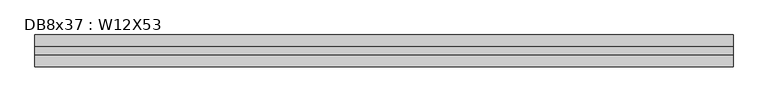
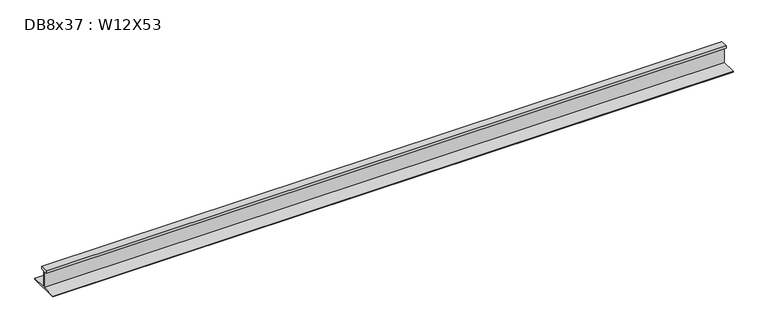
"""IFC4 building model written with IfcOpenShell, lengths in millimetres: beam geometry, DB8x37 : W12X53."""

from ifc_helpers import new_model, si_unit, frame, origin, place, context, project, spatial, polyline, outline, extrude, source, transform, mapped, element, save


def db8x37_w12x53_43f796fb(model_context):
    return source(origin(), model_context, "Body", "SweptSolid", [
        extrude(outline(polyline([(38.1, 145.415), (38.1, 120.015), (2.921, 120.015), (2.921, -48.4505), (152.4, -48.4505), (152.4, -58.1025), (-152.4, -58.1025), (-152.4, -48.4505), (-2.921, -48.4505), (-2.921, 120.015), (-38.1, 120.015), (-38.1, 145.415), (38.1, 145.415)])), frame((-3341.37, 0.0, 0.0), z_axis=(1.0, 0.0, 0.0), x_axis=(0.0, 1.0, 0.0)), (0.0, 0.0, 1.0), 6707.886),
    ])


if __name__ == "__main__":
    model = new_model("IFC4")
    model_context = context("Model", 3, world=origin())
    ifc_project = project(units=[si_unit("LENGTHUNIT", "METRE", prefix="MILLI")], contexts=[model_context])
    site = spatial("IfcSite", under=ifc_project)
    building = spatial("IfcBuilding", under=site)
    placement = place(None, origin())
    db8x37_w12x53_shape = db8x37_w12x53_43f796fb(model_context)
    element("IfcBeam", 1, ObjectType="DB8x37 : W12X53", at=placement, inside=building, context=model_context, shape_type="MappedRepresentation", body=[
        mapped(db8x37_w12x53_shape, transform((0.0, 0.0, 0.0), x_axis=(1.0, 0.0, 0.0), y_axis=(0.0, 1.0, 0.0), z_axis=(0.0, 0.0, 1.0))),
    ])
    save(model, "model.ifc")

# Revit data of these elements
# Type "DB8x37 : W12X53"
#   Assembly Code = "B10"
#   W = 53
#   Length [instance default] = 5' - 0"
#   bf = 0' - 10"
#   d = 1' - 0.1"
#   k = 0' - 1 3/8"
#   k2 = 0' - 0.8"
#   tf = 0' - 0.575"
#   tw = 0' - 0.345"
#   A = 0.108333 SF
#   Structural Material [instance default] = Steel ASTM A992
# Element 1 (IfcBeam, "DB8x37 : W12X53")
#   Materials on its faces: "Steel ASTM A992"
# Materials
#   "Steel ASTM A992": class "Metal", colour RGB 199 199 199, transparency 0, Description = "Structural steel 50ksi", Cost = 0
